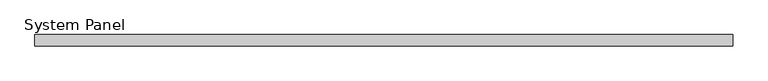
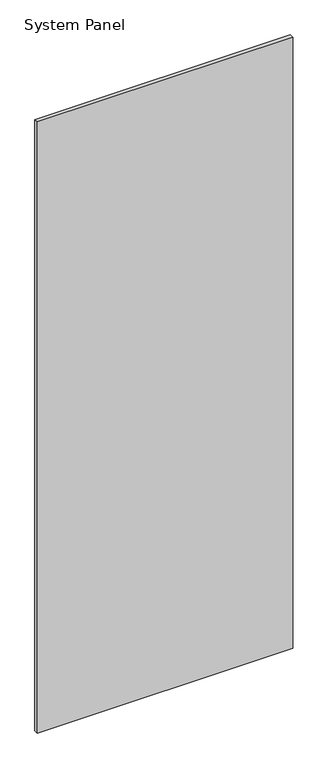
"""IFC4 building model written with IfcOpenShell, lengths in millimetres: plate geometry, System Panel : WWm-Glass-20mm-10mmOffset."""

import ifcopenshell
import ifcopenshell.guid

model = None  # the IFC model being written
_history = None  # IfcOwnerHistory: only IFC2X3 demands one
_inside = {}  # id of a spatial element -> (the spatial element, [elements in it])
_under = {}  # id of a project, library or spatial element -> (it, [spatial elements below it])
_declared = {}  # id of a project -> (the project, [libraries it declares])
_typed = {}  # id of a type object -> (the type object, [elements of that type])
_made_of = {}  # id of a material, layer set ... -> (it, [elements and type objects made of it])


def new_model(schema):
    """Start an empty IFC model of exactly this schema.

    Asked for "IFC4X3", IfcOpenShell would pick the latest addendum, in which some entities
    have other attributes; the version numbers below select the first issue.
    IFC2X3 requires an IfcOwnerHistory on every rooted entity: one is made here for all.
    """
    global model, _history
    if schema == "IFC4X3":
        model = ifcopenshell.file(schema_version=(4, 3, 0, 0))
    else:
        model = ifcopenshell.file(schema=schema)
    _inside.clear()
    _under.clear()
    _declared.clear()
    _typed.clear()
    _made_of.clear()
    _history = None
    if model.schema == "IFC2X3":
        org = make("IfcOrganization", Name="unknown")
        user = make(
            "IfcPersonAndOrganization",
            ThePerson=make("IfcPerson", FamilyName="unknown"),
            TheOrganization=org,
        )
        app = make(
            "IfcApplication",
            ApplicationDeveloper=org,
            Version="unknown",
            ApplicationFullName="unknown",
            ApplicationIdentifier="unknown",
        )
        _history = make(
            "IfcOwnerHistory",
            OwningUser=user,
            OwningApplication=app,
            ChangeAction="ADDED",
            CreationDate=0,
        )
    return model


def make(cls, **values):
    """One entity of the class cls with the attributes given. An attribute that is None is left unset."""
    return model.create_entity(
        cls, **{name: value for name, value in values.items() if value is not None}
    )


def rooted(cls, **values):
    """An entity with a GlobalId (a new one), such as an element, a storey or a relation."""
    return make(cls, GlobalId=ifcopenshell.guid.new(), OwnerHistory=_history, **values)


def si_unit(unit_type, name, prefix=None):
    """IfcSIUnit, for example si_unit("LENGTHUNIT", "METRE", prefix="MILLI")."""
    return make("IfcSIUnit", UnitType=unit_type, Prefix=prefix, Name=name)


def assignment(units):
    """IfcUnitAssignment: the units of a project."""
    return None if units is None else make("IfcUnitAssignment", Units=units)


def point(xyz):
    """IfcCartesianPoint."""
    return None if xyz is None else make("IfcCartesianPoint", Coordinates=xyz)


def direction(xyz):
    """IfcDirection."""
    return None if xyz is None else make("IfcDirection", DirectionRatios=xyz)


def frame(location, z_axis=None, x_axis=None):
    """IfcAxis2Placement3D, a coordinate frame: its origin and axes. An axis left out is left unset."""
    return make(
        "IfcAxis2Placement3D",
        Location=point(location),
        Axis=direction(z_axis),
        RefDirection=direction(x_axis),
    )


def origin():
    """The frame at (0, 0, 0) with its axes left unset."""
    return frame((0.0, 0.0, 0.0))


def origin_with_axes():
    """The frame at (0, 0, 0) with the z axis (0, 0, 1) and the x axis (1, 0, 0) written out."""
    return frame((0.0, 0.0, 0.0), z_axis=(0.0, 0.0, 1.0), x_axis=(1.0, 0.0, 0.0))


def place(relative_to, where):
    """IfcLocalPlacement: puts the frame where relative to a parent placement (None: the world)."""
    return make(
        "IfcLocalPlacement", PlacementRelTo=relative_to, RelativePlacement=where
    )


def context(
    kind, dimensions, precision=None, world=None, true_north=None, identifier=None
):
    """IfcGeometricRepresentationContext, for example the 3D "Model" context."""
    return make(
        "IfcGeometricRepresentationContext",
        ContextIdentifier=identifier,
        ContextType=kind,
        CoordinateSpaceDimension=dimensions,
        Precision=precision,
        WorldCoordinateSystem=world,
        TrueNorth=true_north,
    )


def project(units=None, contexts=None):
    """IfcProject with its units and contexts."""
    return rooted(
        "IfcProject",
        Name="project",
        RepresentationContexts=contexts,
        UnitsInContext=assignment(units),
    )


def spatial(cls, under=None, at=None, **own):
    """A site, building, storey or space (cls), placed at a placement, below another one or the project."""
    s = rooted(cls, ObjectPlacement=at, **own)
    if under is not None:
        _under.setdefault(under.id(), (under, []))[1].append(s)
    return s


def polyline(points):
    """IfcPolyline through the points."""
    return make("IfcPolyline", Points=[point(p) for p in points])


def outline(outer, holes=None, kind="AREA"):
    """IfcArbitraryClosedProfileDef: a profile drawn as a closed curve; with holes, ...WithVoids."""
    if holes is None:
        return make("IfcArbitraryClosedProfileDef", ProfileType=kind, OuterCurve=outer)
    return make(
        "IfcArbitraryProfileDefWithVoids",
        ProfileType=kind,
        OuterCurve=outer,
        InnerCurves=holes,
    )


def extrude(swept, where, along, depth):
    """IfcExtrudedAreaSolid: the profile swept, set in the frame where, extruded along a direction by depth."""
    return make(
        "IfcExtrudedAreaSolid",
        SweptArea=swept,
        Position=where,
        ExtrudedDirection=direction(along),
        Depth=depth,
    )


def shape(context_of_items, identifier, shape_type, items):
    """IfcShapeRepresentation: the items that make up one representation, for example the "Body"."""
    return make(
        "IfcShapeRepresentation",
        ContextOfItems=context_of_items,
        RepresentationIdentifier=identifier,
        RepresentationType=shape_type,
        Items=items,
    )


def source(mapping_origin, context_of_items, identifier, shape_type, items):
    """IfcRepresentationMap: a shape defined once, which mapped items show again and again."""
    return make(
        "IfcRepresentationMap",
        MappingOrigin=mapping_origin,
        MappedRepresentation=shape(context_of_items, identifier, shape_type, items),
    )


def transform(
    local_origin,
    x_axis=None,
    y_axis=None,
    z_axis=None,
    scale=None,
    scale2=None,
    scale3=None,
    uniform=True,
):
    """IfcCartesianTransformationOperator3D, or its non-uniform kind. x_axis, y_axis, z_axis: its Axis1, 2, 3."""
    if uniform:
        return make(
            "IfcCartesianTransformationOperator3D",
            Axis1=direction(x_axis),
            Axis2=direction(y_axis),
            LocalOrigin=point(local_origin),
            Scale=scale,
            Axis3=direction(z_axis),
        )
    return make(
        "IfcCartesianTransformationOperator3DnonUniform",
        Axis1=direction(x_axis),
        Axis2=direction(y_axis),
        LocalOrigin=point(local_origin),
        Scale=scale,
        Axis3=direction(z_axis),
        Scale2=scale2,
        Scale3=scale3,
    )


def mapped(mapping_source, mapping_target):
    """IfcMappedItem: shows the shape of a source again, moved by a transform."""
    return make(
        "IfcMappedItem", MappingSource=mapping_source, MappingTarget=mapping_target
    )


def made_of(thing, what):
    """Note that an element or type object is made of a material, layer set ...; save() writes the relation."""
    if what is not None:
        _made_of.setdefault(what.id(), (what, []))[1].append(thing)
    return thing


def element(
    cls,
    number,
    at=None,
    inside=None,
    cuts=None,
    type_object=None,
    material=None,
    context=None,
    identifier="Body",
    shape_type=None,
    held_by="IfcProductDefinitionShape",
    body=None,
    shapes=None,
    **own,
):
    """One element of the class cls, such as IfcWall. Its Tag is "e" and its number.

    at: its placement. inside: the storey or other place that contains it. cuts: it is an
    opening in that element (IfcRelVoidsElement). A single representation is given by context,
    identifier, shape_type and body (its items); several are given by shapes. held_by: the class
    of the entity that holds the representations. save() writes the other relations.
    """
    e = rooted(cls, Tag="e%d" % number, ObjectPlacement=at, **own)
    if body is not None:
        shapes = [shape(context, identifier, shape_type, body)]
    if shapes is not None:
        e.Representation = make(held_by, Representations=shapes)
    if inside is not None:
        _inside.setdefault(inside.id(), (inside, []))[1].append(e)
    if cuts is not None:
        rooted(
            "IfcRelVoidsElement", RelatingBuildingElement=cuts, RelatedOpeningElement=e
        )
    if type_object is not None:
        _typed.setdefault(type_object.id(), (type_object, []))[1].append(e)
    return made_of(e, material)


def aggregate(whole, parts):
    """IfcRelAggregates: a whole, such as a stair, and the parts it consists of."""
    return rooted("IfcRelAggregates", RelatingObject=whole, RelatedObjects=parts)


def save(model, path):
    """Write the relations noted so far, then the file.

    IfcRelAggregates (storeys below a building ...), IfcRelContainedInSpatialStructure (elements
    in a storey), IfcRelDefinesByType, IfcRelAssociatesMaterial and IfcRelDeclares: one each for
    every whole, place, type object, material and project.
    """
    for whole, parts in _under.values():
        aggregate(whole, parts)
    for where, things in _inside.values():
        rooted(
            "IfcRelContainedInSpatialStructure",
            RelatedElements=things,
            RelatingStructure=where,
        )
    for kind, things in _typed.values():
        rooted("IfcRelDefinesByType", RelatedObjects=things, RelatingType=kind)
    for what, things in _made_of.values():
        rooted("IfcRelAssociatesMaterial", RelatedObjects=things, RelatingMaterial=what)
    for by, libraries in _declared.values():
        rooted("IfcRelDeclares", RelatingContext=by, RelatedDefinitions=libraries)
    model.write(path)


def system_panel_30d55bb6(model_context):
    return source(origin(), model_context, "Body", "SweptSolid", [
        extrude(outline(polyline([(622.8979723, 0.0), (-622.8979723, 0.0), (-622.8979723, 20.0), (622.8979723, 20.0), (622.8979723, 0.0)])), origin_with_axes(), (0.0, 0.0, 1.0), 3150.0),
    ])


if __name__ == "__main__":
    model = new_model("IFC4")
    model_context = context("Model", 3, world=origin())
    ifc_project = project(units=[si_unit("LENGTHUNIT", "METRE", prefix="MILLI")], contexts=[model_context])
    site = spatial("IfcSite", under=ifc_project)
    building = spatial("IfcBuilding", under=site)
    placement = place(None, origin())
    system_panel_shape = system_panel_30d55bb6(model_context)
    element("IfcPlate", 1, ObjectType="System Panel : WWm-Glass-20mm-10mmOffset", at=placement, inside=building, context=model_context, shape_type="MappedRepresentation", body=[
        mapped(system_panel_shape, transform((0.0, 0.0, 0.0), x_axis=(1.0, 0.0, 0.0), y_axis=(0.0, 1.0, 0.0), z_axis=(0.0, 0.0, 1.0))),
    ])
    save(model, "model.ifc")

# Revit data of these elements
# Type "System Panel : WWm-Glass-20mm-10mmOffset"
#   Finish = ""
# Element 1 (IfcPlate, "System Panel : WWm-Glass-20mm-10mmOffset")
#   Materials on its faces: "WW-EC-GL-Storefront"
# Materials
#   "WW-EC-GL-Storefront": class "Glass", colour RGB 236 240 239, transparency 0.85, Description = "Storefront Glass", Cost = 0
